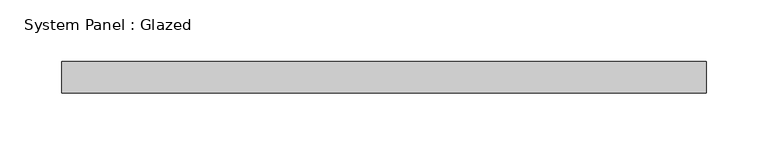
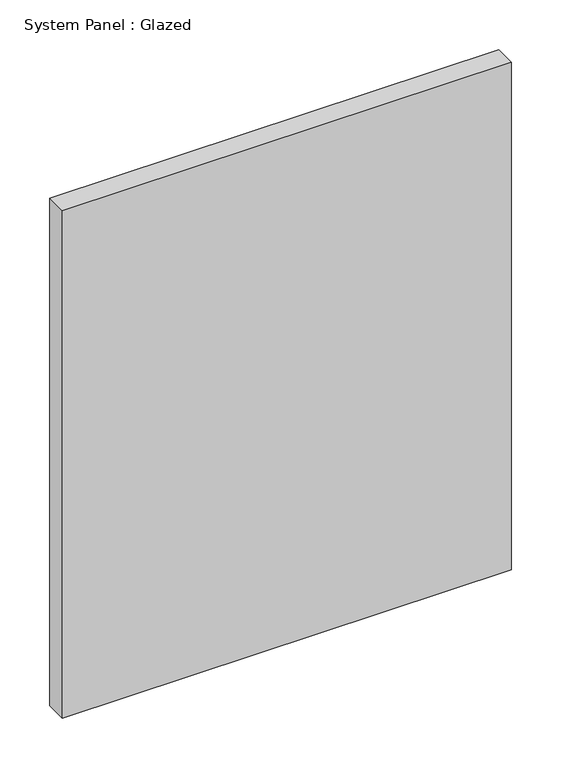
"""IFC4 building model written with IfcOpenShell, lengths in millimetres: plate geometry, System Panel : Glazed."""

from ifc_helpers import new_model, si_unit, origin, origin_with_axes, place, context, project, spatial, polyline, outline, extrude, source, transform, mapped, element, save


def system_panel_glazed_4dcaf286(model_context):
    return source(origin(), model_context, "Body", "SweptSolid", [
        extrude(outline(polyline([(260.35, 19.05), (-260.35, 19.05), (-260.35, 44.45), (260.35, 44.45), (260.35, 19.05)])), origin_with_axes(), (0.0, 0.0, 1.0), 622.3),
    ])


if __name__ == "__main__":
    model = new_model("IFC4")
    model_context = context("Model", 3, world=origin())
    ifc_project = project(units=[si_unit("LENGTHUNIT", "METRE", prefix="MILLI")], contexts=[model_context])
    site = spatial("IfcSite", under=ifc_project)
    building = spatial("IfcBuilding", under=site)
    placement = place(None, origin())
    system_panel_glazed_shape = system_panel_glazed_4dcaf286(model_context)
    element("IfcPlate", 1, ObjectType="System Panel : Glazed", at=placement, inside=building, context=model_context, shape_type="MappedRepresentation", body=[
        mapped(system_panel_glazed_shape, transform((0.0, 0.0, 0.0), x_axis=(1.0, 0.0, 0.0), y_axis=(0.0, 1.0, 0.0), z_axis=(0.0, 0.0, 1.0))),
    ])
    save(model, "model.ifc")

# Revit data of these elements
# Element 1 (IfcPlate, "System Panel : Glazed")
#   Materials on its faces: "Glass"
# Materials
#   "Glass": class "Glass", colour RGB 0 128 192, transparency 0.75
